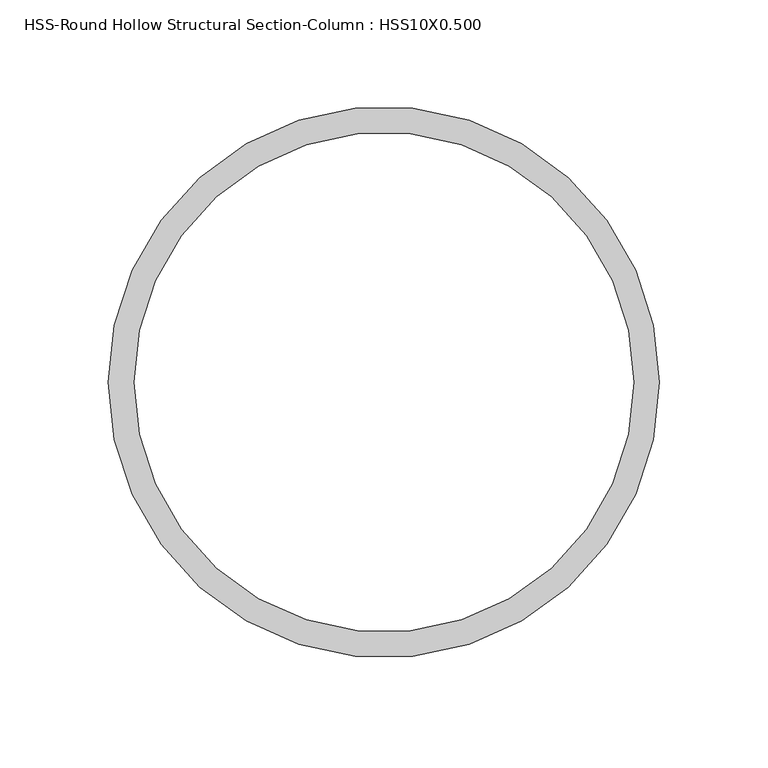
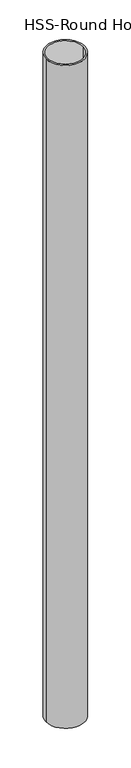
"""IFC4 building model written with IfcOpenShell, lengths in millimetres: column geometry, HSS-Round Hollow Structural Section-Column : HSS10X0.500."""

from ifc_helpers import new_model, si_unit, point, frame, origin, origin_2d, place, context, project, spatial, circle_curve, trimmed, segment, composite_curve, outline, extrude, source, transform, mapped, element, save


def hss_round_hollow_structural_section_column_hss10x0_500_838e436f(model_context):
    return source(origin(), model_context, "Body", "SweptSolid", [
        extrude(outline(composite_curve([segment(trimmed(circle_curve(origin_2d(), 127.0), [point((-127.0, 0.0))], [point((127.0, 0.0))], False, "CARTESIAN"), True, "CONTINUOUS"), segment(trimmed(circle_curve(origin_2d(), 127.0), [point((127.0, 0.0))], [point((-127.0, 0.0))], False, "CARTESIAN"), True, "CONTINUOUS")], self_intersect=False), holes=[composite_curve([segment(trimmed(circle_curve(origin_2d(), 115.189), [point((-115.189, 0.0))], [point((115.189, 0.0))], True, "CARTESIAN"), True, "CONTINUOUS"), segment(trimmed(circle_curve(origin_2d(), 115.189), [point((115.189, 0.0))], [point((-115.189, 0.0))], True, "CARTESIAN"), True, "CONTINUOUS")], self_intersect=False)]), frame((0.0, 0.0, 5969.0), z_axis=(0.0, 0.0, 1.0), x_axis=(1.0, 0.0, 0.0)), (0.0, 0.0, 1.0), 4572.0),
    ])


if __name__ == "__main__":
    model = new_model("IFC4")
    model_context = context("Model", 3, world=origin())
    ifc_project = project(units=[si_unit("LENGTHUNIT", "METRE", prefix="MILLI")], contexts=[model_context])
    site = spatial("IfcSite", under=ifc_project)
    building = spatial("IfcBuilding", under=site)
    placement = place(None, origin())
    hss_round_hollow_structural_section_column_hss10x0_500_shape = hss_round_hollow_structural_section_column_hss10x0_500_838e436f(model_context)
    element("IfcColumn", 1, ObjectType="HSS-Round Hollow Structural Section-Column : HSS10X0.500", at=placement, inside=building, context=model_context, shape_type="MappedRepresentation", body=[
        mapped(hss_round_hollow_structural_section_column_hss10x0_500_shape, transform((0.0, 0.0, 0.0), x_axis=(1.0, 0.0, 0.0), y_axis=(0.0, 1.0, 0.0), z_axis=(0.0, 0.0, 1.0))),
    ])
    save(model, "model.ifc")

# Revit data of these elements
# Type "HSS-Round Hollow Structural Section-Column : HSS10X0.500"
#   Assembly Code = "B10"
#   W = 50.8
#   OD = 0' - 10"
#   t = 0' - 0.465"
#   A = 0.0965278 SF
#   Column Material [instance default] = Metal - Steel - ASTM A53
# Element 1 (IfcColumn, "HSS-Round Hollow Structural Section-Column : HSS10X0.500")
#   Materials on its faces: "Metal - Steel - ASTM A53"
# Materials
#   "Metal - Steel - ASTM A53": class "Metal", colour RGB 128 0 0, transparency 0
